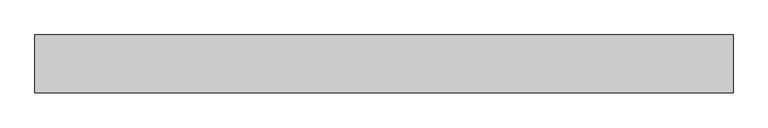
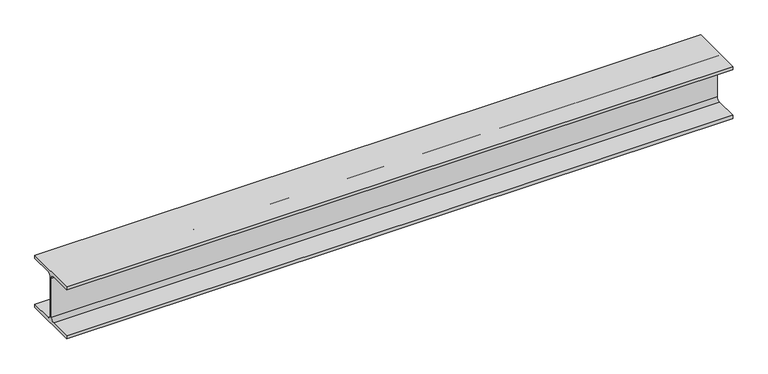
"""IFC4 building model written with IfcOpenShell, lengths in millimetres: beam geometry, 0912_Steel Framing_H-KSD3502 : H_SB_ASB_H-200x200x8x12."""

import ifcopenshell
import ifcopenshell.guid

model = None  # the IFC model being written
_history = None  # IfcOwnerHistory: only IFC2X3 demands one
_inside = {}  # id of a spatial element -> (the spatial element, [elements in it])
_under = {}  # id of a project, library or spatial element -> (it, [spatial elements below it])
_declared = {}  # id of a project -> (the project, [libraries it declares])
_typed = {}  # id of a type object -> (the type object, [elements of that type])
_made_of = {}  # id of a material, layer set ... -> (it, [elements and type objects made of it])


def new_model(schema):
    """Start an empty IFC model of exactly this schema.

    Asked for "IFC4X3", IfcOpenShell would pick the latest addendum, in which some entities
    have other attributes; the version numbers below select the first issue.
    IFC2X3 requires an IfcOwnerHistory on every rooted entity: one is made here for all.
    """
    global model, _history
    if schema == "IFC4X3":
        model = ifcopenshell.file(schema_version=(4, 3, 0, 0))
    else:
        model = ifcopenshell.file(schema=schema)
    _inside.clear()
    _under.clear()
    _declared.clear()
    _typed.clear()
    _made_of.clear()
    _history = None
    if model.schema == "IFC2X3":
        org = make("IfcOrganization", Name="unknown")
        user = make(
            "IfcPersonAndOrganization",
            ThePerson=make("IfcPerson", FamilyName="unknown"),
            TheOrganization=org,
        )
        app = make(
            "IfcApplication",
            ApplicationDeveloper=org,
            Version="unknown",
            ApplicationFullName="unknown",
            ApplicationIdentifier="unknown",
        )
        _history = make(
            "IfcOwnerHistory",
            OwningUser=user,
            OwningApplication=app,
            ChangeAction="ADDED",
            CreationDate=0,
        )
    return model


def make(cls, **values):
    """One entity of the class cls with the attributes given. An attribute that is None is left unset."""
    return model.create_entity(
        cls, **{name: value for name, value in values.items() if value is not None}
    )


def rooted(cls, **values):
    """An entity with a GlobalId (a new one), such as an element, a storey or a relation."""
    return make(cls, GlobalId=ifcopenshell.guid.new(), OwnerHistory=_history, **values)


def si_unit(unit_type, name, prefix=None):
    """IfcSIUnit, for example si_unit("LENGTHUNIT", "METRE", prefix="MILLI")."""
    return make("IfcSIUnit", UnitType=unit_type, Prefix=prefix, Name=name)


def assignment(units):
    """IfcUnitAssignment: the units of a project."""
    return None if units is None else make("IfcUnitAssignment", Units=units)


def point(xyz):
    """IfcCartesianPoint."""
    return None if xyz is None else make("IfcCartesianPoint", Coordinates=xyz)


def direction(xyz):
    """IfcDirection."""
    return None if xyz is None else make("IfcDirection", DirectionRatios=xyz)


def frame(location, z_axis=None, x_axis=None):
    """IfcAxis2Placement3D, a coordinate frame: its origin and axes. An axis left out is left unset."""
    return make(
        "IfcAxis2Placement3D",
        Location=point(location),
        Axis=direction(z_axis),
        RefDirection=direction(x_axis),
    )


def frame_2d(location, x_axis=None):
    """IfcAxis2Placement2D, a coordinate frame in the plane: its origin and x axis."""
    return make(
        "IfcAxis2Placement2D", Location=point(location), RefDirection=direction(x_axis)
    )


def origin():
    """The frame at (0, 0, 0) with its axes left unset."""
    return frame((0.0, 0.0, 0.0))


def place(relative_to, where):
    """IfcLocalPlacement: puts the frame where relative to a parent placement (None: the world)."""
    return make(
        "IfcLocalPlacement", PlacementRelTo=relative_to, RelativePlacement=where
    )


def context(
    kind, dimensions, precision=None, world=None, true_north=None, identifier=None
):
    """IfcGeometricRepresentationContext, for example the 3D "Model" context."""
    return make(
        "IfcGeometricRepresentationContext",
        ContextIdentifier=identifier,
        ContextType=kind,
        CoordinateSpaceDimension=dimensions,
        Precision=precision,
        WorldCoordinateSystem=world,
        TrueNorth=true_north,
    )


def project(units=None, contexts=None):
    """IfcProject with its units and contexts."""
    return rooted(
        "IfcProject",
        Name="project",
        RepresentationContexts=contexts,
        UnitsInContext=assignment(units),
    )


def spatial(cls, under=None, at=None, **own):
    """A site, building, storey or space (cls), placed at a placement, below another one or the project."""
    s = rooted(cls, ObjectPlacement=at, **own)
    if under is not None:
        _under.setdefault(under.id(), (under, []))[1].append(s)
    return s


def polyline(points):
    """IfcPolyline through the points."""
    return make("IfcPolyline", Points=[point(p) for p in points])


def circle_curve(where, radius):
    """IfcCircle in the frame where."""
    return make("IfcCircle", Position=where, Radius=radius)


def trimmed(basis, trim1, trim2, sense, master):
    """IfcTrimmedCurve: the piece of a basis curve between two trims."""
    return make(
        "IfcTrimmedCurve",
        BasisCurve=basis,
        Trim1=trim1,
        Trim2=trim2,
        SenseAgreement=sense,
        MasterRepresentation=master,
    )


def segment(curve, same_sense, transition):
    """IfcCompositeCurveSegment."""
    return make(
        "IfcCompositeCurveSegment",
        Transition=transition,
        SameSense=same_sense,
        ParentCurve=curve,
    )


def composite_curve(segments, self_intersect=None):
    """IfcCompositeCurve: segments joined end to end."""
    return make("IfcCompositeCurve", Segments=segments, SelfIntersect=self_intersect)


def outline(outer, holes=None, kind="AREA"):
    """IfcArbitraryClosedProfileDef: a profile drawn as a closed curve; with holes, ...WithVoids."""
    if holes is None:
        return make("IfcArbitraryClosedProfileDef", ProfileType=kind, OuterCurve=outer)
    return make(
        "IfcArbitraryProfileDefWithVoids",
        ProfileType=kind,
        OuterCurve=outer,
        InnerCurves=holes,
    )


def extrude(swept, where, along, depth):
    """IfcExtrudedAreaSolid: the profile swept, set in the frame where, extruded along a direction by depth."""
    return make(
        "IfcExtrudedAreaSolid",
        SweptArea=swept,
        Position=where,
        ExtrudedDirection=direction(along),
        Depth=depth,
    )


def shape(context_of_items, identifier, shape_type, items):
    """IfcShapeRepresentation: the items that make up one representation, for example the "Body"."""
    return make(
        "IfcShapeRepresentation",
        ContextOfItems=context_of_items,
        RepresentationIdentifier=identifier,
        RepresentationType=shape_type,
        Items=items,
    )


def source(mapping_origin, context_of_items, identifier, shape_type, items):
    """IfcRepresentationMap: a shape defined once, which mapped items show again and again."""
    return make(
        "IfcRepresentationMap",
        MappingOrigin=mapping_origin,
        MappedRepresentation=shape(context_of_items, identifier, shape_type, items),
    )


def transform(
    local_origin,
    x_axis=None,
    y_axis=None,
    z_axis=None,
    scale=None,
    scale2=None,
    scale3=None,
    uniform=True,
):
    """IfcCartesianTransformationOperator3D, or its non-uniform kind. x_axis, y_axis, z_axis: its Axis1, 2, 3."""
    if uniform:
        return make(
            "IfcCartesianTransformationOperator3D",
            Axis1=direction(x_axis),
            Axis2=direction(y_axis),
            LocalOrigin=point(local_origin),
            Scale=scale,
            Axis3=direction(z_axis),
        )
    return make(
        "IfcCartesianTransformationOperator3DnonUniform",
        Axis1=direction(x_axis),
        Axis2=direction(y_axis),
        LocalOrigin=point(local_origin),
        Scale=scale,
        Axis3=direction(z_axis),
        Scale2=scale2,
        Scale3=scale3,
    )


def mapped(mapping_source, mapping_target):
    """IfcMappedItem: shows the shape of a source again, moved by a transform."""
    return make(
        "IfcMappedItem", MappingSource=mapping_source, MappingTarget=mapping_target
    )


def made_of(thing, what):
    """Note that an element or type object is made of a material, layer set ...; save() writes the relation."""
    if what is not None:
        _made_of.setdefault(what.id(), (what, []))[1].append(thing)
    return thing


def element(
    cls,
    number,
    at=None,
    inside=None,
    cuts=None,
    type_object=None,
    material=None,
    context=None,
    identifier="Body",
    shape_type=None,
    held_by="IfcProductDefinitionShape",
    body=None,
    shapes=None,
    **own,
):
    """One element of the class cls, such as IfcWall. Its Tag is "e" and its number.

    at: its placement. inside: the storey or other place that contains it. cuts: it is an
    opening in that element (IfcRelVoidsElement). A single representation is given by context,
    identifier, shape_type and body (its items); several are given by shapes. held_by: the class
    of the entity that holds the representations. save() writes the other relations.
    """
    e = rooted(cls, Tag="e%d" % number, ObjectPlacement=at, **own)
    if body is not None:
        shapes = [shape(context, identifier, shape_type, body)]
    if shapes is not None:
        e.Representation = make(held_by, Representations=shapes)
    if inside is not None:
        _inside.setdefault(inside.id(), (inside, []))[1].append(e)
    if cuts is not None:
        rooted(
            "IfcRelVoidsElement", RelatingBuildingElement=cuts, RelatedOpeningElement=e
        )
    if type_object is not None:
        _typed.setdefault(type_object.id(), (type_object, []))[1].append(e)
    return made_of(e, material)


def aggregate(whole, parts):
    """IfcRelAggregates: a whole, such as a stair, and the parts it consists of."""
    return rooted("IfcRelAggregates", RelatingObject=whole, RelatedObjects=parts)


def save(model, path):
    """Write the relations noted so far, then the file.

    IfcRelAggregates (storeys below a building ...), IfcRelContainedInSpatialStructure (elements
    in a storey), IfcRelDefinesByType, IfcRelAssociatesMaterial and IfcRelDeclares: one each for
    every whole, place, type object, material and project.
    """
    for whole, parts in _under.values():
        aggregate(whole, parts)
    for where, things in _inside.values():
        rooted(
            "IfcRelContainedInSpatialStructure",
            RelatedElements=things,
            RelatingStructure=where,
        )
    for kind, things in _typed.values():
        rooted("IfcRelDefinesByType", RelatedObjects=things, RelatingType=kind)
    for what, things in _made_of.values():
        rooted("IfcRelAssociatesMaterial", RelatedObjects=things, RelatingMaterial=what)
    for by, libraries in _declared.values():
        rooted("IfcRelDeclares", RelatingContext=by, RelatedDefinitions=libraries)
    model.write(path)


def beam_3646a574(model_context):
    return source(origin(), model_context, "Body", "SweptSolid", [
        extrude(outline(composite_curve([segment(polyline([(100.0, -88.0), (100.0, -100.0), (-100.0, -100.0), (-100.0, -88.0), (-17.0, -88.0)]), True, "CONTINUOUS"), segment(trimmed(circle_curve(frame_2d((-17.0, -75.0)), 13.0), [point((-17.0, -88.0))], [point((-4.0, -75.0))], True, "CARTESIAN"), True, "CONTINUOUS"), segment(polyline([(-4.0, -75.0), (-4.0, 75.0)]), True, "CONTINUOUS"), segment(trimmed(circle_curve(frame_2d((-17.0, 75.0)), 13.0), [point((-4.0, 75.0))], [point((-17.0, 88.0))], True, "CARTESIAN"), True, "CONTINUOUS"), segment(polyline([(-17.0, 88.0), (-100.0, 88.0), (-100.0, 100.0), (100.0, 100.0), (100.0, 88.0), (17.0, 88.0)]), True, "CONTINUOUS"), segment(trimmed(circle_curve(frame_2d((17.0, 75.0)), 13.0), [point((17.0, 88.0))], [point((4.0, 75.0))], True, "CARTESIAN"), True, "CONTINUOUS"), segment(polyline([(4.0, 75.0), (4.0, -75.0)]), True, "CONTINUOUS"), segment(trimmed(circle_curve(frame_2d((17.0, -75.0)), 13.0), [point((4.0, -75.0))], [point((17.0, -88.0))], True, "CARTESIAN"), True, "CONTINUOUS"), segment(polyline([(17.0, -88.0), (100.0, -88.0)]), True, "CONTINUOUS")], self_intersect=False)), frame((-1233.7223186, 0.0, 0.0), z_axis=(1.0, 0.0, 0.0), x_axis=(0.0, 1.0, 0.0)), (0.0, 0.0, 1.0), 2418.936364),
    ])


if __name__ == "__main__":
    model = new_model("IFC4")
    model_context = context("Model", 3, world=origin())
    ifc_project = project(units=[si_unit("LENGTHUNIT", "METRE", prefix="MILLI")], contexts=[model_context])
    site = spatial("IfcSite", under=ifc_project)
    building = spatial("IfcBuilding", under=site)
    placement = place(None, origin())
    beam_shape = beam_3646a574(model_context)
    element("IfcBeam", 1, ObjectType="0912_Steel Framing_H-KSD3502 : H_SB_ASB_H-200x200x8x12", at=placement, inside=building, context=model_context, shape_type="MappedRepresentation", body=[
        mapped(beam_shape, transform((0.0, 0.0, 0.0), x_axis=(1.0, 0.0, 0.0), y_axis=(0.0, 1.0, 0.0), z_axis=(0.0, 0.0, 1.0))),
    ])
    save(model, "model.ifc")

# Revit data of these elements
# Type "0912_Steel Framing_H-KSD3502 : H_SB_ASB_H-200x200x8x12"
#   H_WM Code_1 = "S01AA002-00001 | Main Steel Structure Fabrication Work | Shelter/Building | Medium Steel - Standard (90KG/M>Weight≥30KG/M) | Material: (   )"
#   H_WM Code_2 = "S03AA028-00001 | Main Steel Structure Erection Work | Shelter/Building | Medium Steel (90KG/M>Weight≥30KG/M) | Material: (   )"
#   H_WM Code_3 = "S01AA010-00001 | Main Steel Structure Fabrication Work | Shelter/Building | Steel Painting/Coating | for Non-Fireproofed Steel Surface, Surface Preparation, Primer, Second & Final Coat | Material: (   )"
#   H_Q'ty Cal Type Tag = "SB-Q2"
#   Width = 20.0 cm
#   Web Thickness = 0.8 cm
#   Web Fillet = 1.3 cm
#   Warping Constant = 141000.0 cm⁶
#   W = 0
#   Torsional Moment of Inertia = 26.2485 cm⁴
#   Section Area = 63.53 cm²
#   Plastic Modulus weak axis = 244.0 cm³
#   Plastic Modulus strong axis = 525.0 cm³
#   Perimeter = 1.16 m²/m
#   Nominal Weight = 49.90 kgf/m
#   Moment of Inertia weak axis = 1600.00 cm⁴
#   Moment of Inertia strong axis = 4720.00 cm⁴
#   Height = 20.0 cm
#   Flange Thickness = 1.2 cm
#   Elastic Modulus weak axis = 160.0 cm³
#   Elastic Modulus strong axis = 472.0 cm³
#   Centroid Vertical = 10.0 cm
#   Centroid Horizontal = 10.0 cm
#   Ix = 47200000
#   Length [instance default] = 1.5240 m
#   Zx = 525000
#   b = 0.2000 m
#   h = 0.2000 m
#   r = 0.0130 m
#   s = 0.0080 m
#   t = 0.0120 m
#   A = 0.006353 m²
#   Structural Material [instance default] = Steel, 45-345
#   Assembly Code = ""
# Element 1 (IfcBeam, "0912_Steel Framing_H-KSD3502 : H_SB_ASB_H-200x200x8x12")
#   Structural Material = none
# Materials
#   "Steel, 45-345": class "Metal", colour RGB 189 187 185, transparency 0, Description = "Steel 345 MPa", Cost = 0
